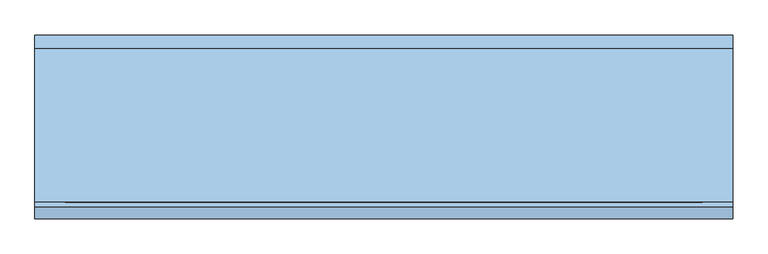
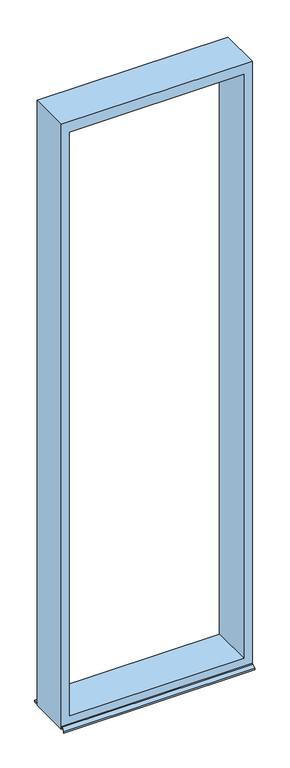
"""IFC4 building model written with IfcOpenShell, lengths in millimetres: window geometry, Fenster - Festverglasung : Feste Verglasung 4.58 x 1.37."""

from ifc_helpers import new_model, si_unit, frame, origin, place, context, project, spatial, polyline, outline, extrude, source, transform, mapped, element, save


def window_2e0b3a34(model_context):
    return source(origin(), model_context, "Body", "SweptSolid", [
        extrude(outline(polyline([(5580.0, 685.0), (5580.0, -685.0), (1000.0, -685.0), (1000.0, 685.0), (5580.0, 685.0)]), holes=[polyline([(5500.0, 625.0), (1080.0, 625.0), (1080.0, -625.0), (5500.0, -625.0), (5500.0, 625.0)])]), frame((0.0, -147.5214598, 0.0), z_axis=(0.0, 1.0, 0.0), x_axis=(0.0, 0.0, 1.0)), (0.0, 0.0, 1.0), 300.0),
        extrude(outline(polyline([(-685.0, 180.0), (685.0, 180.0), (685.0, 152.4785402), (-685.0, 152.4785402), (-685.0, 180.0)])), frame((0.0, 0.0, 1005.0), z_axis=(0.0, 0.0, 1.0), x_axis=(1.0, 0.0, 0.0)), (0.0, 0.0, 1.0), 15.0),
        extrude(outline(polyline([(-157.5436142, 1020.0), (-147.5214598, 1020.0), (-147.5214598, 1018.0), (-157.3455321, 1018.0), (-178.0, 998.3604634), (-178.0, 990.0), (-180.0, 990.0), (-180.0, 1000.0), (-157.5436142, 1020.0)])), frame((-685.0, 0.0, 0.0), z_axis=(1.0, 0.0, 0.0), x_axis=(0.0, 1.0, 0.0)), (0.0, 0.0, 1.0), 1370.0),
    ])


if __name__ == "__main__":
    model = new_model("IFC4")
    model_context = context("Model", 3, world=origin())
    ifc_project = project(units=[si_unit("LENGTHUNIT", "METRE", prefix="MILLI")], contexts=[model_context])
    site = spatial("IfcSite", under=ifc_project)
    building = spatial("IfcBuilding", under=site)
    placement = place(None, origin())
    window_shape = window_2e0b3a34(model_context)
    element("IfcWindow", 1, ObjectType="Fenster - Festverglasung : Feste Verglasung 4.58 x 1.37", at=placement, inside=building, context=model_context, shape_type="MappedRepresentation", body=[
        mapped(window_shape, transform((0.0, 0.0, 0.0), x_axis=(1.0, 0.0, 0.0), y_axis=(0.0, 1.0, 0.0), z_axis=(0.0, 0.0, 1.0))),
    ])
    save(model, "model.ifc")

# Revit data of these elements
# Type "Fenster - Festverglasung : Feste Verglasung 4.58 x 1.37"
#   Type Mark = "59"
#   Operation = "SinglePanel"
#   Keynote = "16.05.01"
#   Visual Light Transmittance = 0.9
#   Solar Heat Gain Coefficient = 0.78
#   Rough Width = 1.370 m
#   Rough Height = 4.580 m
#   Heat Transfer Coefficient (U) = 3.6886 W/(m²·K)
#   Rahmentiefe = 0.300 m
#   Rahmenhöhe unten = 0.080 m
#   Höhe oberer  Rahmen = 0.080 m
#   Rahmenbreite = 0.060 m
#   Height = 4.580 m
#   Einbautiefe (von außen) [instance default] = 0.080 m
#   Width = 1.370 m
#   Wall Closure = 3
#   Bild [instance default] = none
#   Glas [instance default] = none
#   Innere Fensterbank [instance default] = none
#   Äußere Fensterbank [instance default] = none
#   Construction Type Id = ""
#   Analytic Construction = (empty or 0)
# Element 1 (IfcWindow, "Fenster - Festverglasung : Feste Verglasung 4.58 x 1.37")
#   Einbautiefe (von außen) = 0.002479 m
#   Materials on its faces: "Kunststoff - Weiß", "Holz - Birke"
# Materials
#   "Kunststoff - Weiß": class "Kunststoff", colour RGB 249 249 249, transparency 0, Cost = 0
#   "Holz - Birke": class "Holz", colour RGB 213 164 103, transparency 0, Cost = 0
